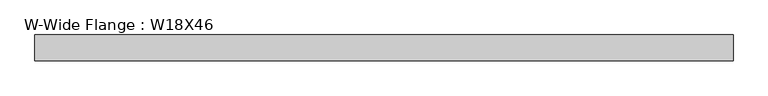
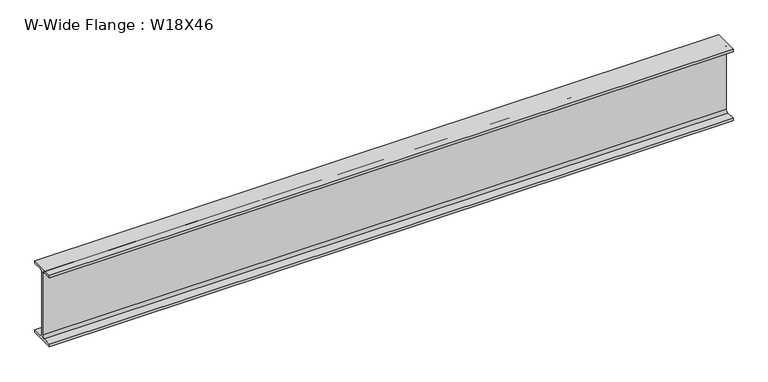
"""IFC4 building model written with IfcOpenShell, lengths in millimetres: beam geometry, W-Wide Flange : W18X46."""

from ifc_helpers import new_model, si_unit, point, frame, frame_2d, origin, place, context, project, spatial, polyline, circle_curve, trimmed, segment, composite_curve, outline, extrude, source, transform, mapped, element, save


def w_wide_flange_w18x46_b43e2ba2(model_context):
    return source(origin(), model_context, "Body", "SweptSolid", [
        extrude(outline(composite_curve([segment(polyline([(76.962, -214.503), (76.962, -229.87), (-76.962, -229.87), (-76.962, -214.503), (-20.955, -214.503)]), True, "CONTINUOUS"), segment(trimmed(circle_curve(frame_2d((-20.955, -198.12)), 16.383), [point((-20.955, -214.503))], [point((-4.572, -198.12))], True, "CARTESIAN"), True, "CONTINUOUS"), segment(polyline([(-4.572, -198.12), (-4.572, 198.12)]), True, "CONTINUOUS"), segment(trimmed(circle_curve(frame_2d((-20.955, 198.12)), 16.383), [point((-4.572, 198.12))], [point((-20.955, 214.503))], True, "CARTESIAN"), True, "CONTINUOUS"), segment(polyline([(-20.955, 214.503), (-76.962, 214.503), (-76.962, 229.87), (76.962, 229.87), (76.962, 214.503), (20.955, 214.503)]), True, "CONTINUOUS"), segment(trimmed(circle_curve(frame_2d((20.955, 198.12)), 16.383), [point((20.955, 214.503))], [point((4.572, 198.12))], True, "CARTESIAN"), True, "CONTINUOUS"), segment(polyline([(4.572, 198.12), (4.572, -198.12)]), True, "CONTINUOUS"), segment(trimmed(circle_curve(frame_2d((20.955, -198.12)), 16.383), [point((4.572, -198.12))], [point((20.955, -214.503))], True, "CARTESIAN"), True, "CONTINUOUS"), segment(polyline([(20.955, -214.503), (76.962, -214.503)]), True, "CONTINUOUS")], self_intersect=False)), frame((-2082.8, 0.0, 0.0), z_axis=(1.0, 0.0, 0.0), x_axis=(0.0, 1.0, 0.0)), (0.0, 0.0, 1.0), 4165.6),
    ])


if __name__ == "__main__":
    model = new_model("IFC4")
    model_context = context("Model", 3, world=origin())
    ifc_project = project(units=[si_unit("LENGTHUNIT", "METRE", prefix="MILLI")], contexts=[model_context])
    site = spatial("IfcSite", under=ifc_project)
    building = spatial("IfcBuilding", under=site)
    placement = place(None, origin())
    w_wide_flange_w18x46_shape = w_wide_flange_w18x46_b43e2ba2(model_context)
    element("IfcBeam", 1, ObjectType="W-Wide Flange : W18X46", at=placement, inside=building, context=model_context, shape_type="MappedRepresentation", body=[
        mapped(w_wide_flange_w18x46_shape, transform((0.0, 0.0, 0.0), x_axis=(1.0, 0.0, 0.0), y_axis=(0.0, 1.0, 0.0), z_axis=(0.0, 0.0, 1.0))),
    ])
    save(model, "model.ifc")

# Revit data of these elements
# Type "W-Wide Flange : W18X46"
#   Assembly Code = "B10"
#   W = 46
#   Length [instance default] = 5' - 0"
#   bf = 0' - 6.06"
#   d = 1' - 6.1"
#   k = 0' - 1 1/4"
#   k2 = 0' - 0.645"
#   tf = 0' - 0.605"
#   tw = 0' - 0.36"
#   A = 0.09375 SF
#   Structural Material [instance default] = Steel ASTM A992
# Element 1 (IfcBeam, "W-Wide Flange : W18X46")
#   Materials on its faces: "Steel ASTM A992"
# Materials
#   "Steel ASTM A992": class "Metal", colour RGB 199 199 199, transparency 0, Description = "Structural steel 50ksi", Cost = 0
